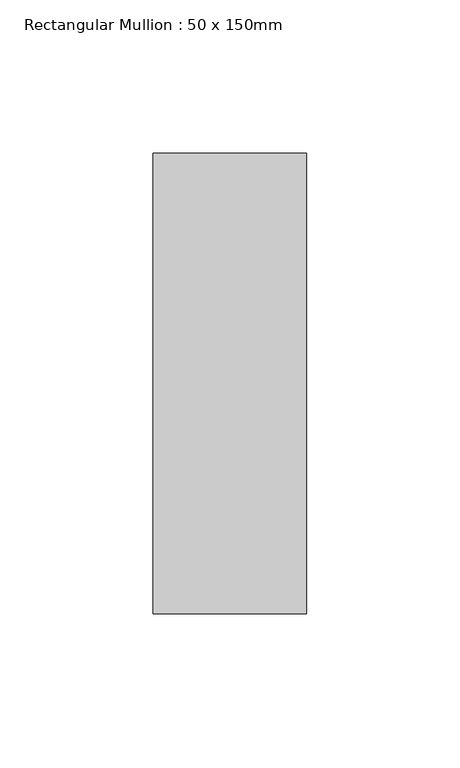
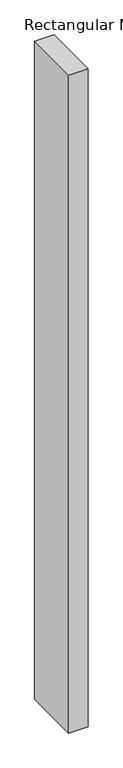
"""IFC4 building model written with IfcOpenShell, lengths in millimetres: member geometry, Rectangular Mullion : 50 x 150mm."""

from ifc_helpers import new_model, si_unit, frame, origin, place, context, project, spatial, polyline, outline, extrude, source, transform, mapped, element, save


def rectangular_mullion_50_x_150mm_da41d874(model_context):
    return source(origin(), model_context, "Body", "SweptSolid", [
        extrude(outline(polyline([(25.0, 75.0), (25.0, -75.0), (-25.0, -75.0), (-25.0, 75.0), (25.0, 75.0)])), frame((0.0, 0.0, -1775.8970067), z_axis=(0.0, 0.0, 1.0), x_axis=(1.0, 0.0, 0.0)), (0.0, 0.0, 1.0), 1775.8970067),
    ])


if __name__ == "__main__":
    model = new_model("IFC4")
    model_context = context("Model", 3, world=origin())
    ifc_project = project(units=[si_unit("LENGTHUNIT", "METRE", prefix="MILLI")], contexts=[model_context])
    site = spatial("IfcSite", under=ifc_project)
    building = spatial("IfcBuilding", under=site)
    placement = place(None, origin())
    rectangular_mullion_50_x_150mm_shape = rectangular_mullion_50_x_150mm_da41d874(model_context)
    element("IfcMember", 1, ObjectType="Rectangular Mullion : 50 x 150mm", at=placement, inside=building, context=model_context, shape_type="MappedRepresentation", body=[
        mapped(rectangular_mullion_50_x_150mm_shape, transform((0.0, 0.0, 0.0), x_axis=(1.0, 0.0, 0.0), y_axis=(0.0, 1.0, 0.0), z_axis=(0.0, 0.0, 1.0))),
    ])
    save(model, "model.ifc")

# Revit data of these elements
# Type "Rectangular Mullion : 50 x 150mm"
#   Keynote = "H11"
#   built-in parameter 1007304 = 0.492126 (stored number, unit not read)
#   built-in parameter 1007301 = 0.082021 (stored number, unit not read)
#   built-in parameter 1007300 = 0.082021 (stored number, unit not read)
# Element 1 (IfcMember, "Rectangular Mullion : 50 x 150mm")
#   Materials on its faces: "Aluminium"
# Materials
#   "Aluminium": class "Metal", colour RGB 247 247 247, transparency 0, Description = "Aluminium 6061", Cost = 0
